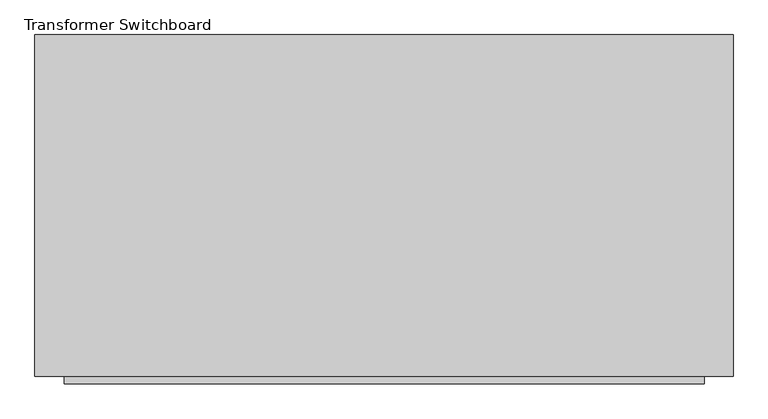
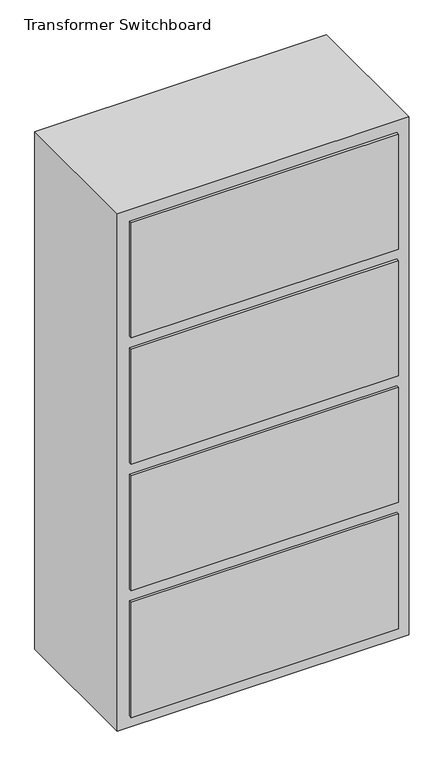
"""IFC4 building model written with IfcOpenShell, lengths in millimetres: proxy geometry, Transformer Switchboard."""

from ifc_helpers import new_model, si_unit, frame, origin, origin_with_axes, place, context, project, spatial, polyline, outline, extrude, source, transform, mapped, element, save


def transformer_switchboard_4d195b30(model_context):
    return source(origin(), model_context, "Body", "SweptSolid", [
        extrude(outline(polyline([(558.8, -609.6), (-558.8, -609.6), (-558.8, -596.9), (558.8, -596.9), (558.8, -609.6)])), frame((0.0, 0.0, 1727.2), z_axis=(0.0, 0.0, 1.0), x_axis=(1.0, 0.0, 0.0)), (0.0, 0.0, 1.0), 508.0),
        extrude(outline(polyline([(558.8, -609.6), (-558.8, -609.6), (-558.8, -596.9), (558.8, -596.9), (558.8, -609.6)])), frame((0.0, 0.0, 1168.4), z_axis=(0.0, 0.0, 1.0), x_axis=(1.0, 0.0, 0.0)), (0.0, 0.0, 1.0), 508.0),
        extrude(outline(polyline([(558.8, -609.6), (-558.8, -609.6), (-558.8, -596.9), (558.8, -596.9), (558.8, -609.6)])), frame((0.0, 0.0, 609.6), z_axis=(0.0, 0.0, 1.0), x_axis=(1.0, 0.0, 0.0)), (0.0, 0.0, 1.0), 508.0),
        extrude(outline(polyline([(558.8, -609.6), (-558.8, -609.6), (-558.8, -596.9), (558.8, -596.9), (558.8, -609.6)])), frame((0.0, 0.0, 50.8), z_axis=(0.0, 0.0, 1.0), x_axis=(1.0, 0.0, 0.0)), (0.0, 0.0, 1.0), 508.0),
        extrude(outline(polyline([(609.6, 0.0), (609.6, -596.9), (-609.6, -596.9), (-609.6, 0.0), (609.6, 0.0)])), origin_with_axes(), (0.0, 0.0, 1.0), 2286.0),
    ])


if __name__ == "__main__":
    model = new_model("IFC4")
    model_context = context("Model", 3, world=origin())
    ifc_project = project(units=[si_unit("LENGTHUNIT", "METRE", prefix="MILLI")], contexts=[model_context])
    site = spatial("IfcSite", under=ifc_project)
    building = spatial("IfcBuilding", under=site)
    placement = place(None, origin())
    transformer_switchboard_shape = transformer_switchboard_4d195b30(model_context)
    element("IfcBuildingElementProxy", 1, Name="Transformer Switchboard : 24\"deep x 48\" wide x 90\"H", ObjectType="Transformer Switchboard : 24\"deep x 48\" wide x 90\"H", at=placement, inside=building, context=model_context, shape_type="MappedRepresentation", body=[
        mapped(transformer_switchboard_shape, transform((0.0, 0.0, 0.0), x_axis=(1.0, 0.0, 0.0), y_axis=(0.0, 1.0, 0.0), z_axis=(0.0, 0.0, 1.0))),
    ])
    save(model, "model.ifc")

# Revit data of these elements
# Type "Transformer Switchboard : 24\"deep x 48\" wide x 90\"H"
#   Switchboard Width = 2' - 0"
#   Switchboard Length = 4' - 0"
#   Switchboard Height = 7' - 6"
#   Primary Voltage = 480 V
#   Panel Length = 3' - 8"
#   Panel Height = 1' - 8"
#   Length 1 = 4' - 0"
#   Height 1 = 7' - 6"
#   Half Switchboard Length = 2' - 0"
#   Clearance_Side_Back = 2' - 0"
#   Clearance_Front = 5' - 0"
#   Primary Number of Poles = 3
#   Switchboard Material = none
#   Load Classification = Other
